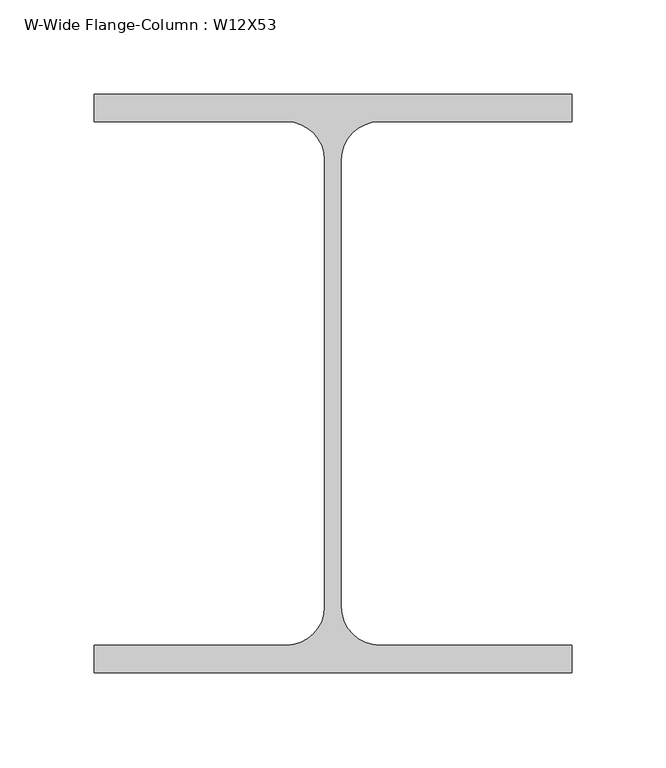
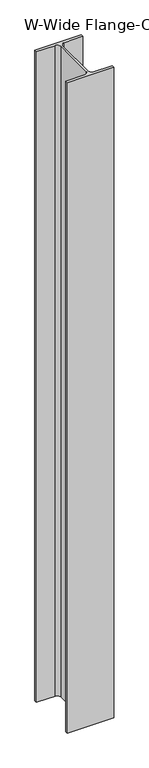
"""IFC4 building model written with IfcOpenShell, lengths in millimetres: column geometry, W-Wide Flange-Column : W12X53."""

import ifcopenshell
import ifcopenshell.guid

model = None  # the IFC model being written
_history = None  # IfcOwnerHistory: only IFC2X3 demands one
_inside = {}  # id of a spatial element -> (the spatial element, [elements in it])
_under = {}  # id of a project, library or spatial element -> (it, [spatial elements below it])
_declared = {}  # id of a project -> (the project, [libraries it declares])
_typed = {}  # id of a type object -> (the type object, [elements of that type])
_made_of = {}  # id of a material, layer set ... -> (it, [elements and type objects made of it])


def new_model(schema):
    """Start an empty IFC model of exactly this schema.

    Asked for "IFC4X3", IfcOpenShell would pick the latest addendum, in which some entities
    have other attributes; the version numbers below select the first issue.
    IFC2X3 requires an IfcOwnerHistory on every rooted entity: one is made here for all.
    """
    global model, _history
    if schema == "IFC4X3":
        model = ifcopenshell.file(schema_version=(4, 3, 0, 0))
    else:
        model = ifcopenshell.file(schema=schema)
    _inside.clear()
    _under.clear()
    _declared.clear()
    _typed.clear()
    _made_of.clear()
    _history = None
    if model.schema == "IFC2X3":
        org = make("IfcOrganization", Name="unknown")
        user = make(
            "IfcPersonAndOrganization",
            ThePerson=make("IfcPerson", FamilyName="unknown"),
            TheOrganization=org,
        )
        app = make(
            "IfcApplication",
            ApplicationDeveloper=org,
            Version="unknown",
            ApplicationFullName="unknown",
            ApplicationIdentifier="unknown",
        )
        _history = make(
            "IfcOwnerHistory",
            OwningUser=user,
            OwningApplication=app,
            ChangeAction="ADDED",
            CreationDate=0,
        )
    return model


def make(cls, **values):
    """One entity of the class cls with the attributes given. An attribute that is None is left unset."""
    return model.create_entity(
        cls, **{name: value for name, value in values.items() if value is not None}
    )


def rooted(cls, **values):
    """An entity with a GlobalId (a new one), such as an element, a storey or a relation."""
    return make(cls, GlobalId=ifcopenshell.guid.new(), OwnerHistory=_history, **values)


def si_unit(unit_type, name, prefix=None):
    """IfcSIUnit, for example si_unit("LENGTHUNIT", "METRE", prefix="MILLI")."""
    return make("IfcSIUnit", UnitType=unit_type, Prefix=prefix, Name=name)


def assignment(units):
    """IfcUnitAssignment: the units of a project."""
    return None if units is None else make("IfcUnitAssignment", Units=units)


def point(xyz):
    """IfcCartesianPoint."""
    return None if xyz is None else make("IfcCartesianPoint", Coordinates=xyz)


def direction(xyz):
    """IfcDirection."""
    return None if xyz is None else make("IfcDirection", DirectionRatios=xyz)


def frame(location, z_axis=None, x_axis=None):
    """IfcAxis2Placement3D, a coordinate frame: its origin and axes. An axis left out is left unset."""
    return make(
        "IfcAxis2Placement3D",
        Location=point(location),
        Axis=direction(z_axis),
        RefDirection=direction(x_axis),
    )


def frame_2d(location, x_axis=None):
    """IfcAxis2Placement2D, a coordinate frame in the plane: its origin and x axis."""
    return make(
        "IfcAxis2Placement2D", Location=point(location), RefDirection=direction(x_axis)
    )


def origin():
    """The frame at (0, 0, 0) with its axes left unset."""
    return frame((0.0, 0.0, 0.0))


def place(relative_to, where):
    """IfcLocalPlacement: puts the frame where relative to a parent placement (None: the world)."""
    return make(
        "IfcLocalPlacement", PlacementRelTo=relative_to, RelativePlacement=where
    )


def context(
    kind, dimensions, precision=None, world=None, true_north=None, identifier=None
):
    """IfcGeometricRepresentationContext, for example the 3D "Model" context."""
    return make(
        "IfcGeometricRepresentationContext",
        ContextIdentifier=identifier,
        ContextType=kind,
        CoordinateSpaceDimension=dimensions,
        Precision=precision,
        WorldCoordinateSystem=world,
        TrueNorth=true_north,
    )


def project(units=None, contexts=None):
    """IfcProject with its units and contexts."""
    return rooted(
        "IfcProject",
        Name="project",
        RepresentationContexts=contexts,
        UnitsInContext=assignment(units),
    )


def spatial(cls, under=None, at=None, **own):
    """A site, building, storey or space (cls), placed at a placement, below another one or the project."""
    s = rooted(cls, ObjectPlacement=at, **own)
    if under is not None:
        _under.setdefault(under.id(), (under, []))[1].append(s)
    return s


def polyline(points):
    """IfcPolyline through the points."""
    return make("IfcPolyline", Points=[point(p) for p in points])


def circle_curve(where, radius):
    """IfcCircle in the frame where."""
    return make("IfcCircle", Position=where, Radius=radius)


def trimmed(basis, trim1, trim2, sense, master):
    """IfcTrimmedCurve: the piece of a basis curve between two trims."""
    return make(
        "IfcTrimmedCurve",
        BasisCurve=basis,
        Trim1=trim1,
        Trim2=trim2,
        SenseAgreement=sense,
        MasterRepresentation=master,
    )


def segment(curve, same_sense, transition):
    """IfcCompositeCurveSegment."""
    return make(
        "IfcCompositeCurveSegment",
        Transition=transition,
        SameSense=same_sense,
        ParentCurve=curve,
    )


def composite_curve(segments, self_intersect=None):
    """IfcCompositeCurve: segments joined end to end."""
    return make("IfcCompositeCurve", Segments=segments, SelfIntersect=self_intersect)


def outline(outer, holes=None, kind="AREA"):
    """IfcArbitraryClosedProfileDef: a profile drawn as a closed curve; with holes, ...WithVoids."""
    if holes is None:
        return make("IfcArbitraryClosedProfileDef", ProfileType=kind, OuterCurve=outer)
    return make(
        "IfcArbitraryProfileDefWithVoids",
        ProfileType=kind,
        OuterCurve=outer,
        InnerCurves=holes,
    )


def extrude(swept, where, along, depth):
    """IfcExtrudedAreaSolid: the profile swept, set in the frame where, extruded along a direction by depth."""
    return make(
        "IfcExtrudedAreaSolid",
        SweptArea=swept,
        Position=where,
        ExtrudedDirection=direction(along),
        Depth=depth,
    )


def shape(context_of_items, identifier, shape_type, items):
    """IfcShapeRepresentation: the items that make up one representation, for example the "Body"."""
    return make(
        "IfcShapeRepresentation",
        ContextOfItems=context_of_items,
        RepresentationIdentifier=identifier,
        RepresentationType=shape_type,
        Items=items,
    )


def source(mapping_origin, context_of_items, identifier, shape_type, items):
    """IfcRepresentationMap: a shape defined once, which mapped items show again and again."""
    return make(
        "IfcRepresentationMap",
        MappingOrigin=mapping_origin,
        MappedRepresentation=shape(context_of_items, identifier, shape_type, items),
    )


def transform(
    local_origin,
    x_axis=None,
    y_axis=None,
    z_axis=None,
    scale=None,
    scale2=None,
    scale3=None,
    uniform=True,
):
    """IfcCartesianTransformationOperator3D, or its non-uniform kind. x_axis, y_axis, z_axis: its Axis1, 2, 3."""
    if uniform:
        return make(
            "IfcCartesianTransformationOperator3D",
            Axis1=direction(x_axis),
            Axis2=direction(y_axis),
            LocalOrigin=point(local_origin),
            Scale=scale,
            Axis3=direction(z_axis),
        )
    return make(
        "IfcCartesianTransformationOperator3DnonUniform",
        Axis1=direction(x_axis),
        Axis2=direction(y_axis),
        LocalOrigin=point(local_origin),
        Scale=scale,
        Axis3=direction(z_axis),
        Scale2=scale2,
        Scale3=scale3,
    )


def mapped(mapping_source, mapping_target):
    """IfcMappedItem: shows the shape of a source again, moved by a transform."""
    return make(
        "IfcMappedItem", MappingSource=mapping_source, MappingTarget=mapping_target
    )


def made_of(thing, what):
    """Note that an element or type object is made of a material, layer set ...; save() writes the relation."""
    if what is not None:
        _made_of.setdefault(what.id(), (what, []))[1].append(thing)
    return thing


def element(
    cls,
    number,
    at=None,
    inside=None,
    cuts=None,
    type_object=None,
    material=None,
    context=None,
    identifier="Body",
    shape_type=None,
    held_by="IfcProductDefinitionShape",
    body=None,
    shapes=None,
    **own,
):
    """One element of the class cls, such as IfcWall. Its Tag is "e" and its number.

    at: its placement. inside: the storey or other place that contains it. cuts: it is an
    opening in that element (IfcRelVoidsElement). A single representation is given by context,
    identifier, shape_type and body (its items); several are given by shapes. held_by: the class
    of the entity that holds the representations. save() writes the other relations.
    """
    e = rooted(cls, Tag="e%d" % number, ObjectPlacement=at, **own)
    if body is not None:
        shapes = [shape(context, identifier, shape_type, body)]
    if shapes is not None:
        e.Representation = make(held_by, Representations=shapes)
    if inside is not None:
        _inside.setdefault(inside.id(), (inside, []))[1].append(e)
    if cuts is not None:
        rooted(
            "IfcRelVoidsElement", RelatingBuildingElement=cuts, RelatedOpeningElement=e
        )
    if type_object is not None:
        _typed.setdefault(type_object.id(), (type_object, []))[1].append(e)
    return made_of(e, material)


def aggregate(whole, parts):
    """IfcRelAggregates: a whole, such as a stair, and the parts it consists of."""
    return rooted("IfcRelAggregates", RelatingObject=whole, RelatedObjects=parts)


def save(model, path):
    """Write the relations noted so far, then the file.

    IfcRelAggregates (storeys below a building ...), IfcRelContainedInSpatialStructure (elements
    in a storey), IfcRelDefinesByType, IfcRelAssociatesMaterial and IfcRelDeclares: one each for
    every whole, place, type object, material and project.
    """
    for whole, parts in _under.values():
        aggregate(whole, parts)
    for where, things in _inside.values():
        rooted(
            "IfcRelContainedInSpatialStructure",
            RelatedElements=things,
            RelatingStructure=where,
        )
    for kind, things in _typed.values():
        rooted("IfcRelDefinesByType", RelatedObjects=things, RelatingType=kind)
    for what, things in _made_of.values():
        rooted("IfcRelAssociatesMaterial", RelatedObjects=things, RelatingMaterial=what)
    for by, libraries in _declared.values():
        rooted("IfcRelDeclares", RelatingContext=by, RelatedDefinitions=libraries)
    model.write(path)


def w_wide_flange_column_w12x53_e48874d2(model_context):
    return source(origin(), model_context, "Body", "SweptSolid", [
        extrude(outline(composite_curve([segment(polyline([(127.0, 153.67), (127.0, 139.065), (24.7015, 139.065)]), True, "CONTINUOUS"), segment(trimmed(circle_curve(frame_2d((24.7015, 118.745)), 20.32), [point((24.7015, 139.065))], [point((4.3815, 118.745))], True, "CARTESIAN"), True, "CONTINUOUS"), segment(polyline([(4.3815, 118.745), (4.3815, -118.745)]), True, "CONTINUOUS"), segment(trimmed(circle_curve(frame_2d((24.7015, -118.745)), 20.32), [point((4.3815, -118.745))], [point((24.7015, -139.065))], True, "CARTESIAN"), True, "CONTINUOUS"), segment(polyline([(24.7015, -139.065), (127.0, -139.065), (127.0, -153.67), (-127.0, -153.67), (-127.0, -139.065), (-24.7015, -139.065)]), True, "CONTINUOUS"), segment(trimmed(circle_curve(frame_2d((-24.7015, -118.745)), 20.32), [point((-24.7015, -139.065))], [point((-4.3815, -118.745))], True, "CARTESIAN"), True, "CONTINUOUS"), segment(polyline([(-4.3815, -118.745), (-4.3815, 118.745)]), True, "CONTINUOUS"), segment(trimmed(circle_curve(frame_2d((-24.7015, 118.745)), 20.32), [point((-4.3815, 118.745))], [point((-24.7015, 139.065))], True, "CARTESIAN"), True, "CONTINUOUS"), segment(polyline([(-24.7015, 139.065), (-127.0, 139.065), (-127.0, 153.67), (127.0, 153.67)]), True, "CONTINUOUS")], self_intersect=False)), frame((0.0, 0.0, 8655.05), z_axis=(0.0, 0.0, 1.0), x_axis=(1.0, 0.0, 0.0)), (0.0, 0.0, 1.0), 3752.85),
    ])


if __name__ == "__main__":
    model = new_model("IFC4")
    model_context = context("Model", 3, world=origin())
    ifc_project = project(units=[si_unit("LENGTHUNIT", "METRE", prefix="MILLI")], contexts=[model_context])
    site = spatial("IfcSite", under=ifc_project)
    building = spatial("IfcBuilding", under=site)
    placement = place(None, origin())
    w_wide_flange_column_w12x53_shape = w_wide_flange_column_w12x53_e48874d2(model_context)
    element("IfcColumn", 1, ObjectType="W-Wide Flange-Column : W12X53", at=placement, inside=building, context=model_context, shape_type="MappedRepresentation", body=[
        mapped(w_wide_flange_column_w12x53_shape, transform((0.0, 0.0, 0.0), x_axis=(1.0, 0.0, 0.0), y_axis=(0.0, 1.0, 0.0), z_axis=(0.0, 0.0, 1.0))),
    ])
    save(model, "model.ifc")

# Revit data of these elements
# Type "W-Wide Flange-Column : W12X53"
#   Assembly Code = "B10"
#   W = 53
#   bf = 0' - 10"
#   d = 1' - 0.1"
#   k = 0' - 1 3/8"
#   kr = 0' - 0.8"
#   tf = 0' - 0.575"
#   tw = 0' - 0.345"
#   A = 0.108333 SF
#   Structural Material [instance default] = Steel ASTM A992
# Element 1 (IfcColumn, "W-Wide Flange-Column : W12X53")
#   Materials on its faces: "Steel ASTM A992"
# Materials
#   "Steel ASTM A992": class "Metal", colour RGB 199 199 199, transparency 0, Description = "Structural steel 50ksi", Cost = 0
